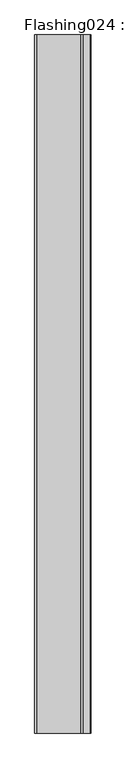
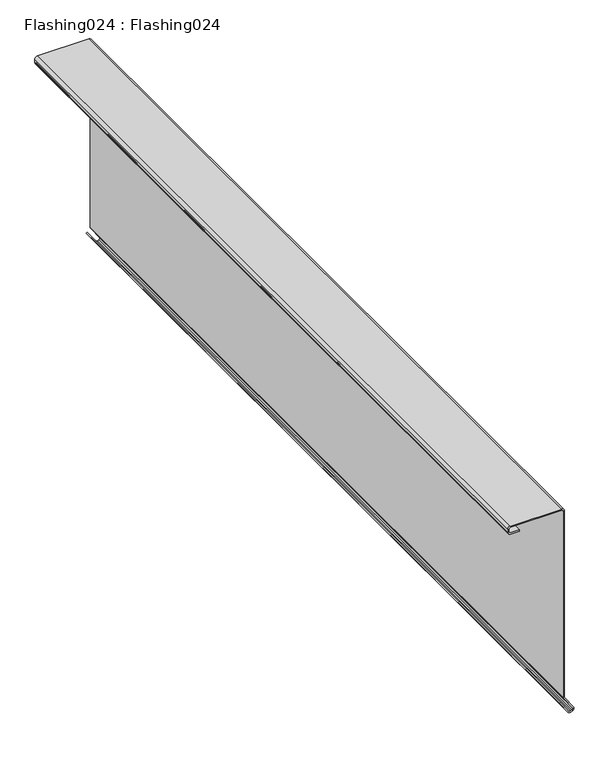
"""IFC4 building model written with IfcOpenShell, lengths in millimetres: proxy geometry, Flashing024 : Flashing024."""

import ifcopenshell
import ifcopenshell.guid

model = None  # the IFC model being written
_history = None  # IfcOwnerHistory: only IFC2X3 demands one
_inside = {}  # id of a spatial element -> (the spatial element, [elements in it])
_under = {}  # id of a project, library or spatial element -> (it, [spatial elements below it])
_declared = {}  # id of a project -> (the project, [libraries it declares])
_typed = {}  # id of a type object -> (the type object, [elements of that type])
_made_of = {}  # id of a material, layer set ... -> (it, [elements and type objects made of it])


def new_model(schema):
    """Start an empty IFC model of exactly this schema.

    Asked for "IFC4X3", IfcOpenShell would pick the latest addendum, in which some entities
    have other attributes; the version numbers below select the first issue.
    IFC2X3 requires an IfcOwnerHistory on every rooted entity: one is made here for all.
    """
    global model, _history
    if schema == "IFC4X3":
        model = ifcopenshell.file(schema_version=(4, 3, 0, 0))
    else:
        model = ifcopenshell.file(schema=schema)
    _inside.clear()
    _under.clear()
    _declared.clear()
    _typed.clear()
    _made_of.clear()
    _history = None
    if model.schema == "IFC2X3":
        org = make("IfcOrganization", Name="unknown")
        user = make(
            "IfcPersonAndOrganization",
            ThePerson=make("IfcPerson", FamilyName="unknown"),
            TheOrganization=org,
        )
        app = make(
            "IfcApplication",
            ApplicationDeveloper=org,
            Version="unknown",
            ApplicationFullName="unknown",
            ApplicationIdentifier="unknown",
        )
        _history = make(
            "IfcOwnerHistory",
            OwningUser=user,
            OwningApplication=app,
            ChangeAction="ADDED",
            CreationDate=0,
        )
    return model


def make(cls, **values):
    """One entity of the class cls with the attributes given. An attribute that is None is left unset."""
    return model.create_entity(
        cls, **{name: value for name, value in values.items() if value is not None}
    )


def rooted(cls, **values):
    """An entity with a GlobalId (a new one), such as an element, a storey or a relation."""
    return make(cls, GlobalId=ifcopenshell.guid.new(), OwnerHistory=_history, **values)


def si_unit(unit_type, name, prefix=None):
    """IfcSIUnit, for example si_unit("LENGTHUNIT", "METRE", prefix="MILLI")."""
    return make("IfcSIUnit", UnitType=unit_type, Prefix=prefix, Name=name)


def assignment(units):
    """IfcUnitAssignment: the units of a project."""
    return None if units is None else make("IfcUnitAssignment", Units=units)


def point(xyz):
    """IfcCartesianPoint."""
    return None if xyz is None else make("IfcCartesianPoint", Coordinates=xyz)


def direction(xyz):
    """IfcDirection."""
    return None if xyz is None else make("IfcDirection", DirectionRatios=xyz)


def frame(location, z_axis=None, x_axis=None):
    """IfcAxis2Placement3D, a coordinate frame: its origin and axes. An axis left out is left unset."""
    return make(
        "IfcAxis2Placement3D",
        Location=point(location),
        Axis=direction(z_axis),
        RefDirection=direction(x_axis),
    )


def frame_2d(location, x_axis=None):
    """IfcAxis2Placement2D, a coordinate frame in the plane: its origin and x axis."""
    return make(
        "IfcAxis2Placement2D", Location=point(location), RefDirection=direction(x_axis)
    )


def origin():
    """The frame at (0, 0, 0) with its axes left unset."""
    return frame((0.0, 0.0, 0.0))


def place(relative_to, where):
    """IfcLocalPlacement: puts the frame where relative to a parent placement (None: the world)."""
    return make(
        "IfcLocalPlacement", PlacementRelTo=relative_to, RelativePlacement=where
    )


def context(
    kind, dimensions, precision=None, world=None, true_north=None, identifier=None
):
    """IfcGeometricRepresentationContext, for example the 3D "Model" context."""
    return make(
        "IfcGeometricRepresentationContext",
        ContextIdentifier=identifier,
        ContextType=kind,
        CoordinateSpaceDimension=dimensions,
        Precision=precision,
        WorldCoordinateSystem=world,
        TrueNorth=true_north,
    )


def project(units=None, contexts=None):
    """IfcProject with its units and contexts."""
    return rooted(
        "IfcProject",
        Name="project",
        RepresentationContexts=contexts,
        UnitsInContext=assignment(units),
    )


def spatial(cls, under=None, at=None, **own):
    """A site, building, storey or space (cls), placed at a placement, below another one or the project."""
    s = rooted(cls, ObjectPlacement=at, **own)
    if under is not None:
        _under.setdefault(under.id(), (under, []))[1].append(s)
    return s


def polyline(points):
    """IfcPolyline through the points."""
    return make("IfcPolyline", Points=[point(p) for p in points])


def circle_curve(where, radius):
    """IfcCircle in the frame where."""
    return make("IfcCircle", Position=where, Radius=radius)


def trimmed(basis, trim1, trim2, sense, master):
    """IfcTrimmedCurve: the piece of a basis curve between two trims."""
    return make(
        "IfcTrimmedCurve",
        BasisCurve=basis,
        Trim1=trim1,
        Trim2=trim2,
        SenseAgreement=sense,
        MasterRepresentation=master,
    )


def segment(curve, same_sense, transition):
    """IfcCompositeCurveSegment."""
    return make(
        "IfcCompositeCurveSegment",
        Transition=transition,
        SameSense=same_sense,
        ParentCurve=curve,
    )


def composite_curve(segments, self_intersect=None):
    """IfcCompositeCurve: segments joined end to end."""
    return make("IfcCompositeCurve", Segments=segments, SelfIntersect=self_intersect)


def outline(outer, holes=None, kind="AREA"):
    """IfcArbitraryClosedProfileDef: a profile drawn as a closed curve; with holes, ...WithVoids."""
    if holes is None:
        return make("IfcArbitraryClosedProfileDef", ProfileType=kind, OuterCurve=outer)
    return make(
        "IfcArbitraryProfileDefWithVoids",
        ProfileType=kind,
        OuterCurve=outer,
        InnerCurves=holes,
    )


def extrude(swept, where, along, depth):
    """IfcExtrudedAreaSolid: the profile swept, set in the frame where, extruded along a direction by depth."""
    return make(
        "IfcExtrudedAreaSolid",
        SweptArea=swept,
        Position=where,
        ExtrudedDirection=direction(along),
        Depth=depth,
    )


def shape(context_of_items, identifier, shape_type, items):
    """IfcShapeRepresentation: the items that make up one representation, for example the "Body"."""
    return make(
        "IfcShapeRepresentation",
        ContextOfItems=context_of_items,
        RepresentationIdentifier=identifier,
        RepresentationType=shape_type,
        Items=items,
    )


def source(mapping_origin, context_of_items, identifier, shape_type, items):
    """IfcRepresentationMap: a shape defined once, which mapped items show again and again."""
    return make(
        "IfcRepresentationMap",
        MappingOrigin=mapping_origin,
        MappedRepresentation=shape(context_of_items, identifier, shape_type, items),
    )


def transform(
    local_origin,
    x_axis=None,
    y_axis=None,
    z_axis=None,
    scale=None,
    scale2=None,
    scale3=None,
    uniform=True,
):
    """IfcCartesianTransformationOperator3D, or its non-uniform kind. x_axis, y_axis, z_axis: its Axis1, 2, 3."""
    if uniform:
        return make(
            "IfcCartesianTransformationOperator3D",
            Axis1=direction(x_axis),
            Axis2=direction(y_axis),
            LocalOrigin=point(local_origin),
            Scale=scale,
            Axis3=direction(z_axis),
        )
    return make(
        "IfcCartesianTransformationOperator3DnonUniform",
        Axis1=direction(x_axis),
        Axis2=direction(y_axis),
        LocalOrigin=point(local_origin),
        Scale=scale,
        Axis3=direction(z_axis),
        Scale2=scale2,
        Scale3=scale3,
    )


def mapped(mapping_source, mapping_target):
    """IfcMappedItem: shows the shape of a source again, moved by a transform."""
    return make(
        "IfcMappedItem", MappingSource=mapping_source, MappingTarget=mapping_target
    )


def made_of(thing, what):
    """Note that an element or type object is made of a material, layer set ...; save() writes the relation."""
    if what is not None:
        _made_of.setdefault(what.id(), (what, []))[1].append(thing)
    return thing


def element(
    cls,
    number,
    at=None,
    inside=None,
    cuts=None,
    type_object=None,
    material=None,
    context=None,
    identifier="Body",
    shape_type=None,
    held_by="IfcProductDefinitionShape",
    body=None,
    shapes=None,
    **own,
):
    """One element of the class cls, such as IfcWall. Its Tag is "e" and its number.

    at: its placement. inside: the storey or other place that contains it. cuts: it is an
    opening in that element (IfcRelVoidsElement). A single representation is given by context,
    identifier, shape_type and body (its items); several are given by shapes. held_by: the class
    of the entity that holds the representations. save() writes the other relations.
    """
    e = rooted(cls, Tag="e%d" % number, ObjectPlacement=at, **own)
    if body is not None:
        shapes = [shape(context, identifier, shape_type, body)]
    if shapes is not None:
        e.Representation = make(held_by, Representations=shapes)
    if inside is not None:
        _inside.setdefault(inside.id(), (inside, []))[1].append(e)
    if cuts is not None:
        rooted(
            "IfcRelVoidsElement", RelatingBuildingElement=cuts, RelatedOpeningElement=e
        )
    if type_object is not None:
        _typed.setdefault(type_object.id(), (type_object, []))[1].append(e)
    return made_of(e, material)


def aggregate(whole, parts):
    """IfcRelAggregates: a whole, such as a stair, and the parts it consists of."""
    return rooted("IfcRelAggregates", RelatingObject=whole, RelatedObjects=parts)


def save(model, path):
    """Write the relations noted so far, then the file.

    IfcRelAggregates (storeys below a building ...), IfcRelContainedInSpatialStructure (elements
    in a storey), IfcRelDefinesByType, IfcRelAssociatesMaterial and IfcRelDeclares: one each for
    every whole, place, type object, material and project.
    """
    for whole, parts in _under.values():
        aggregate(whole, parts)
    for where, things in _inside.values():
        rooted(
            "IfcRelContainedInSpatialStructure",
            RelatedElements=things,
            RelatingStructure=where,
        )
    for kind, things in _typed.values():
        rooted("IfcRelDefinesByType", RelatedObjects=things, RelatingType=kind)
    for what, things in _made_of.values():
        rooted("IfcRelAssociatesMaterial", RelatedObjects=things, RelatingMaterial=what)
    for by, libraries in _declared.values():
        rooted("IfcRelDeclares", RelatingContext=by, RelatedDefinitions=libraries)
    model.write(path)


def flashing024_flashing024_9ad17ddb(model_context):
    return source(origin(), model_context, "Body", "SweptSolid", [
        extrude(outline(composite_curve([segment(trimmed(circle_curve(frame_2d((41323.8783762, 6183.9556944)), 6.35), [point((41320.2092308, 6178.7730434))], [point((41318.4012804, 6187.1687804))], False, "CARTESIAN"), True, "CONTINUOUS"), segment(polyline([(41318.4012804, 6187.1687804), (41320.1425067, 6190.1369125)]), True, "CONTINUOUS"), segment(trimmed(circle_curve(frame_2d((41325.6196026, 6186.9238265)), 6.35), [point((41320.1425067, 6190.1369125))], [point((41329.2370767, 6192.1426751))], False, "CARTESIAN"), True, "CONTINUOUS"), segment(polyline([(41329.2370767, 6192.1426751), (41359.2301171, 6171.3528311)]), True, "CONTINUOUS"), segment(trimmed(circle_curve(frame_2d((41362.8475913, 6176.5716797)), 6.35), [point((41359.2301171, 6171.3528311))], [point((41362.8475913, 6170.2216797))], True, "CARTESIAN"), True, "CONTINUOUS"), segment(polyline([(41362.8475913, 6170.2216797), (41842.9189039, 6170.2216797)]), True, "CONTINUOUS"), segment(trimmed(circle_curve(frame_2d((41842.9189039, 6163.8716797)), 6.35), [point((41842.9189039, 6170.2216797))], [point((41849.2689039, 6163.8716797))], False, "CARTESIAN"), True, "CONTINUOUS"), segment(polyline([(41849.2689039, 6163.8716797), (41849.2689039, 6038.1540605)]), True, "CONTINUOUS"), segment(trimmed(circle_curve(frame_2d((41842.9189039, 6038.1540605)), 6.35), [point((41849.2689039, 6038.1540605))], [point((41842.9189039, 6031.8040605))], False, "CARTESIAN"), True, "CONTINUOUS"), segment(polyline([(41842.9189039, 6031.8040605), (41835.0524976, 6031.8040605)]), True, "CONTINUOUS"), segment(trimmed(circle_curve(frame_2d((41835.0524976, 6038.1540605)), 6.35), [point((41835.0524976, 6031.8040605))], [point((41828.7024976, 6038.1540605))], False, "CARTESIAN"), True, "CONTINUOUS"), segment(polyline([(41828.7024976, 6038.1540605), (41828.7024976, 6060.1805253), (41831.7024976, 6060.1805253), (41831.7024976, 6038.1540605)]), True, "CONTINUOUS"), segment(trimmed(circle_curve(frame_2d((41835.0524976, 6038.1540605)), 3.35), [point((41831.7024976, 6038.1540605))], [point((41835.0524976, 6034.8040605))], True, "CARTESIAN"), True, "CONTINUOUS"), segment(polyline([(41835.0524976, 6034.8040605), (41842.9189039, 6034.8040605)]), True, "CONTINUOUS"), segment(trimmed(circle_curve(frame_2d((41842.9189039, 6038.1540605)), 3.35), [point((41842.9189039, 6034.8040605))], [point((41846.2689039, 6038.1540605))], True, "CARTESIAN"), True, "CONTINUOUS"), segment(polyline([(41846.2689039, 6038.1540605), (41846.2689039, 6163.8716797)]), True, "CONTINUOUS"), segment(trimmed(circle_curve(frame_2d((41842.9189039, 6163.8716797)), 3.35), [point((41846.2689039, 6163.8716797))], [point((41842.9189039, 6167.2216797))], True, "CARTESIAN"), True, "CONTINUOUS"), segment(polyline([(41842.9189039, 6167.2216797), (41362.8475913, 6167.2216797)]), True, "CONTINUOUS"), segment(trimmed(circle_curve(frame_2d((41362.8475913, 6176.5716797)), 9.35), [point((41362.8475913, 6167.2216797))], [point((41357.5210742, 6168.8872333))], False, "CARTESIAN"), True, "CONTINUOUS"), segment(polyline([(41357.5210742, 6168.8872333), (41327.5280338, 6189.6770774)]), True, "CONTINUOUS"), segment(trimmed(circle_curve(frame_2d((41325.6196026, 6186.9238265)), 3.35), [point((41327.5280338, 6189.6770774))], [point((41322.730111, 6188.6189191))], True, "CARTESIAN"), True, "CONTINUOUS"), segment(polyline([(41322.730111, 6188.6189191), (41320.9888847, 6185.650787)]), True, "CONTINUOUS"), segment(trimmed(circle_curve(frame_2d((41323.8783762, 6183.9556944)), 3.35), [point((41320.9888847, 6185.650787))], [point((41321.9426853, 6181.2215399))], True, "CARTESIAN"), True, "CONTINUOUS"), segment(polyline([(41321.9426853, 6181.2215399), (41352.3883692, 6159.6670035), (41350.6549147, 6157.218507), (41320.2092308, 6178.7730434)]), True, "CONTINUOUS")], self_intersect=False)), frame((0.0, 2217.3609988, 0.0), z_axis=(0.0, 1.0, 0.0), x_axis=(0.0, 0.0, 1.0)), (0.0, 0.0, 1.0), 2000.0),
    ])


if __name__ == "__main__":
    model = new_model("IFC4")
    model_context = context("Model", 3, world=origin())
    ifc_project = project(units=[si_unit("LENGTHUNIT", "METRE", prefix="MILLI")], contexts=[model_context])
    site = spatial("IfcSite", under=ifc_project)
    building = spatial("IfcBuilding", under=site)
    placement = place(None, origin())
    flashing024_flashing024_shape = flashing024_flashing024_9ad17ddb(model_context)
    element("IfcBuildingElementProxy", 1, Name="Flashing024 : Flashing024", ObjectType="Flashing024 : Flashing024", at=placement, inside=building, context=model_context, shape_type="MappedRepresentation", body=[
        mapped(flashing024_flashing024_shape, transform((0.0, 0.0, 0.0), x_axis=(1.0, 0.0, 0.0), y_axis=(0.0, 1.0, 0.0), z_axis=(0.0, 0.0, 1.0))),
    ])
    save(model, "model.ifc")

# Revit data of these elements
# Type "Flashing024 : Flashing024"
#   NameOverride = "Flashing024"
# Element 1 (IfcBuildingElementProxy, "Flashing024 : Flashing024")
#   Materials on its faces: "BRAKE METAL EAVE TRIM TO MATCH STANDING SEAM COLOR"
# Materials
#   "BRAKE METAL EAVE TRIM TO MATCH STANDING SEAM COLOR": class "Unassigned", colour RGB 128 128 128, transparency 0, Cost = 0
